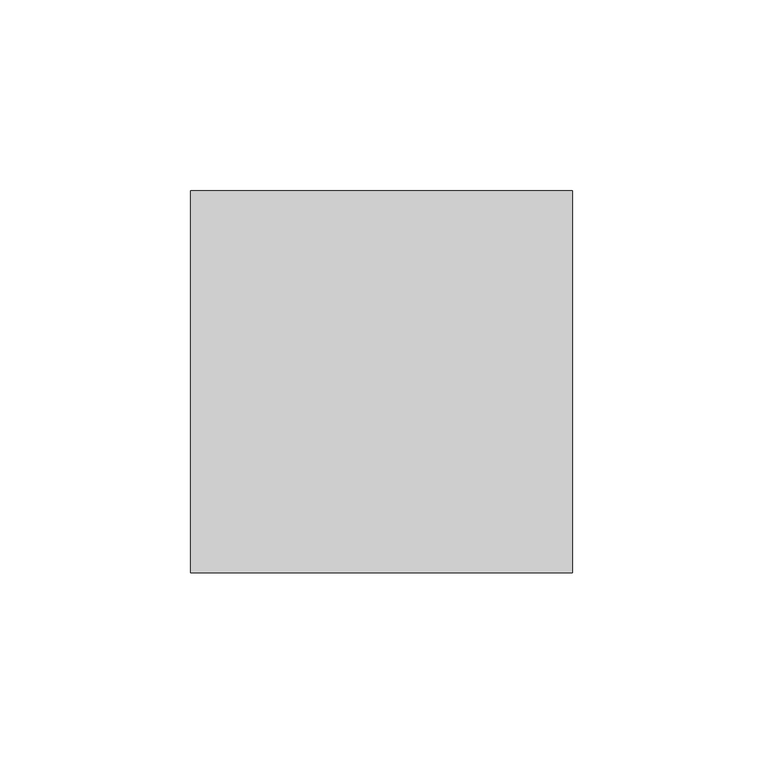
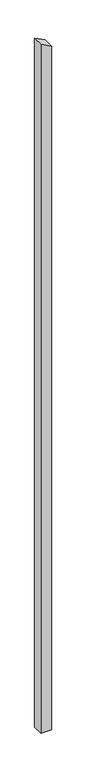
"""IFC4 building model written with IfcOpenShell, lengths in millimetres: column geometry, Holzstütze 159406 : Holzstütze 159406."""

import ifcopenshell
import ifcopenshell.guid

model = None  # the IFC model being written
_history = None  # IfcOwnerHistory: only IFC2X3 demands one
_inside = {}  # id of a spatial element -> (the spatial element, [elements in it])
_under = {}  # id of a project, library or spatial element -> (it, [spatial elements below it])
_declared = {}  # id of a project -> (the project, [libraries it declares])
_typed = {}  # id of a type object -> (the type object, [elements of that type])
_made_of = {}  # id of a material, layer set ... -> (it, [elements and type objects made of it])


def new_model(schema):
    """Start an empty IFC model of exactly this schema.

    Asked for "IFC4X3", IfcOpenShell would pick the latest addendum, in which some entities
    have other attributes; the version numbers below select the first issue.
    IFC2X3 requires an IfcOwnerHistory on every rooted entity: one is made here for all.
    """
    global model, _history
    if schema == "IFC4X3":
        model = ifcopenshell.file(schema_version=(4, 3, 0, 0))
    else:
        model = ifcopenshell.file(schema=schema)
    _inside.clear()
    _under.clear()
    _declared.clear()
    _typed.clear()
    _made_of.clear()
    _history = None
    if model.schema == "IFC2X3":
        org = make("IfcOrganization", Name="unknown")
        user = make(
            "IfcPersonAndOrganization",
            ThePerson=make("IfcPerson", FamilyName="unknown"),
            TheOrganization=org,
        )
        app = make(
            "IfcApplication",
            ApplicationDeveloper=org,
            Version="unknown",
            ApplicationFullName="unknown",
            ApplicationIdentifier="unknown",
        )
        _history = make(
            "IfcOwnerHistory",
            OwningUser=user,
            OwningApplication=app,
            ChangeAction="ADDED",
            CreationDate=0,
        )
    return model


def make(cls, **values):
    """One entity of the class cls with the attributes given. An attribute that is None is left unset."""
    return model.create_entity(
        cls, **{name: value for name, value in values.items() if value is not None}
    )


def rooted(cls, **values):
    """An entity with a GlobalId (a new one), such as an element, a storey or a relation."""
    return make(cls, GlobalId=ifcopenshell.guid.new(), OwnerHistory=_history, **values)


def si_unit(unit_type, name, prefix=None):
    """IfcSIUnit, for example si_unit("LENGTHUNIT", "METRE", prefix="MILLI")."""
    return make("IfcSIUnit", UnitType=unit_type, Prefix=prefix, Name=name)


def assignment(units):
    """IfcUnitAssignment: the units of a project."""
    return None if units is None else make("IfcUnitAssignment", Units=units)


def point(xyz):
    """IfcCartesianPoint."""
    return None if xyz is None else make("IfcCartesianPoint", Coordinates=xyz)


def direction(xyz):
    """IfcDirection."""
    return None if xyz is None else make("IfcDirection", DirectionRatios=xyz)


def frame(location, z_axis=None, x_axis=None):
    """IfcAxis2Placement3D, a coordinate frame: its origin and axes. An axis left out is left unset."""
    return make(
        "IfcAxis2Placement3D",
        Location=point(location),
        Axis=direction(z_axis),
        RefDirection=direction(x_axis),
    )


def origin():
    """The frame at (0, 0, 0) with its axes left unset."""
    return frame((0.0, 0.0, 0.0))


def place(relative_to, where):
    """IfcLocalPlacement: puts the frame where relative to a parent placement (None: the world)."""
    return make(
        "IfcLocalPlacement", PlacementRelTo=relative_to, RelativePlacement=where
    )


def context(
    kind, dimensions, precision=None, world=None, true_north=None, identifier=None
):
    """IfcGeometricRepresentationContext, for example the 3D "Model" context."""
    return make(
        "IfcGeometricRepresentationContext",
        ContextIdentifier=identifier,
        ContextType=kind,
        CoordinateSpaceDimension=dimensions,
        Precision=precision,
        WorldCoordinateSystem=world,
        TrueNorth=true_north,
    )


def project(units=None, contexts=None):
    """IfcProject with its units and contexts."""
    return rooted(
        "IfcProject",
        Name="project",
        RepresentationContexts=contexts,
        UnitsInContext=assignment(units),
    )


def spatial(cls, under=None, at=None, **own):
    """A site, building, storey or space (cls), placed at a placement, below another one or the project."""
    s = rooted(cls, ObjectPlacement=at, **own)
    if under is not None:
        _under.setdefault(under.id(), (under, []))[1].append(s)
    return s


def polyline(points):
    """IfcPolyline through the points."""
    return make("IfcPolyline", Points=[point(p) for p in points])


def outline(outer, holes=None, kind="AREA"):
    """IfcArbitraryClosedProfileDef: a profile drawn as a closed curve; with holes, ...WithVoids."""
    if holes is None:
        return make("IfcArbitraryClosedProfileDef", ProfileType=kind, OuterCurve=outer)
    return make(
        "IfcArbitraryProfileDefWithVoids",
        ProfileType=kind,
        OuterCurve=outer,
        InnerCurves=holes,
    )


def extrude(swept, where, along, depth):
    """IfcExtrudedAreaSolid: the profile swept, set in the frame where, extruded along a direction by depth."""
    return make(
        "IfcExtrudedAreaSolid",
        SweptArea=swept,
        Position=where,
        ExtrudedDirection=direction(along),
        Depth=depth,
    )


def shape(context_of_items, identifier, shape_type, items):
    """IfcShapeRepresentation: the items that make up one representation, for example the "Body"."""
    return make(
        "IfcShapeRepresentation",
        ContextOfItems=context_of_items,
        RepresentationIdentifier=identifier,
        RepresentationType=shape_type,
        Items=items,
    )


def source(mapping_origin, context_of_items, identifier, shape_type, items):
    """IfcRepresentationMap: a shape defined once, which mapped items show again and again."""
    return make(
        "IfcRepresentationMap",
        MappingOrigin=mapping_origin,
        MappedRepresentation=shape(context_of_items, identifier, shape_type, items),
    )


def transform(
    local_origin,
    x_axis=None,
    y_axis=None,
    z_axis=None,
    scale=None,
    scale2=None,
    scale3=None,
    uniform=True,
):
    """IfcCartesianTransformationOperator3D, or its non-uniform kind. x_axis, y_axis, z_axis: its Axis1, 2, 3."""
    if uniform:
        return make(
            "IfcCartesianTransformationOperator3D",
            Axis1=direction(x_axis),
            Axis2=direction(y_axis),
            LocalOrigin=point(local_origin),
            Scale=scale,
            Axis3=direction(z_axis),
        )
    return make(
        "IfcCartesianTransformationOperator3DnonUniform",
        Axis1=direction(x_axis),
        Axis2=direction(y_axis),
        LocalOrigin=point(local_origin),
        Scale=scale,
        Axis3=direction(z_axis),
        Scale2=scale2,
        Scale3=scale3,
    )


def mapped(mapping_source, mapping_target):
    """IfcMappedItem: shows the shape of a source again, moved by a transform."""
    return make(
        "IfcMappedItem", MappingSource=mapping_source, MappingTarget=mapping_target
    )


def made_of(thing, what):
    """Note that an element or type object is made of a material, layer set ...; save() writes the relation."""
    if what is not None:
        _made_of.setdefault(what.id(), (what, []))[1].append(thing)
    return thing


def element(
    cls,
    number,
    at=None,
    inside=None,
    cuts=None,
    type_object=None,
    material=None,
    context=None,
    identifier="Body",
    shape_type=None,
    held_by="IfcProductDefinitionShape",
    body=None,
    shapes=None,
    **own,
):
    """One element of the class cls, such as IfcWall. Its Tag is "e" and its number.

    at: its placement. inside: the storey or other place that contains it. cuts: it is an
    opening in that element (IfcRelVoidsElement). A single representation is given by context,
    identifier, shape_type and body (its items); several are given by shapes. held_by: the class
    of the entity that holds the representations. save() writes the other relations.
    """
    e = rooted(cls, Tag="e%d" % number, ObjectPlacement=at, **own)
    if body is not None:
        shapes = [shape(context, identifier, shape_type, body)]
    if shapes is not None:
        e.Representation = make(held_by, Representations=shapes)
    if inside is not None:
        _inside.setdefault(inside.id(), (inside, []))[1].append(e)
    if cuts is not None:
        rooted(
            "IfcRelVoidsElement", RelatingBuildingElement=cuts, RelatedOpeningElement=e
        )
    if type_object is not None:
        _typed.setdefault(type_object.id(), (type_object, []))[1].append(e)
    return made_of(e, material)


def aggregate(whole, parts):
    """IfcRelAggregates: a whole, such as a stair, and the parts it consists of."""
    return rooted("IfcRelAggregates", RelatingObject=whole, RelatedObjects=parts)


def save(model, path):
    """Write the relations noted so far, then the file.

    IfcRelAggregates (storeys below a building ...), IfcRelContainedInSpatialStructure (elements
    in a storey), IfcRelDefinesByType, IfcRelAssociatesMaterial and IfcRelDeclares: one each for
    every whole, place, type object, material and project.
    """
    for whole, parts in _under.values():
        aggregate(whole, parts)
    for where, things in _inside.values():
        rooted(
            "IfcRelContainedInSpatialStructure",
            RelatedElements=things,
            RelatingStructure=where,
        )
    for kind, things in _typed.values():
        rooted("IfcRelDefinesByType", RelatedObjects=things, RelatingType=kind)
    for what, things in _made_of.values():
        rooted("IfcRelAssociatesMaterial", RelatedObjects=things, RelatingMaterial=what)
    for by, libraries in _declared.values():
        rooted("IfcRelDeclares", RelatingContext=by, RelatedDefinitions=libraries)
    model.write(path)


def column_ac924ca4(model_context):
    return source(origin(), model_context, "Body", "SweptSolid", [
        extrude(outline(polyline([(-500.0, 174197.7593015), (-500.0, 174297.7593015), (6345.7118258, 174297.7593015), (6396.6643707, 174197.7593015), (-500.0, 174197.7593015)])), frame((0.0, 44151.7297978, 0.0), z_axis=(0.0, 1.0, 0.0), x_axis=(0.0, 0.0, 1.0)), (0.0, 0.0, 1.0), 100.0),
    ])


if __name__ == "__main__":
    model = new_model("IFC4")
    model_context = context("Model", 3, world=origin())
    ifc_project = project(units=[si_unit("LENGTHUNIT", "METRE", prefix="MILLI")], contexts=[model_context])
    site = spatial("IfcSite", under=ifc_project)
    building = spatial("IfcBuilding", under=site)
    placement = place(None, origin())
    column_shape = column_ac924ca4(model_context)
    element("IfcColumn", 1, ObjectType="Holzstütze 159406 : Holzstütze 159406", at=placement, inside=building, context=model_context, shape_type="MappedRepresentation", body=[
        mapped(column_shape, transform((0.0, 0.0, 0.0), x_axis=(1.0, 0.0, 0.0), y_axis=(0.0, 1.0, 0.0), z_axis=(0.0, 0.0, 1.0))),
    ])
    save(model, "model.ifc")

# Revit data of these elements
# Type "Holzstütze 159406 : Holzstütze 159406"
#   Abrechnungsart = "m"
#   Allright_Bauteil_ID = "0152St 0000143354"
#   Bezeichnung = "Holzstütze"
#   Codetext = "ST-HOLZ\\"
#   Gewerk = "Zimmer- und Holzbauarbeiten"
#   Material = "Holz"
#   Objektname = "Stütze"
#   NameOverride = "Holzstütze"
#   Reference = "Holzstütze"
#   Status = "NEW"
#   ThermalTransmittance = 0.0000 BTU/(h·ft²·°F)
#   Roll = 0.00°
#   Slope = 0.00°
#   2D Interaktion = yes
#   IsExternal = yes
#   LoadBearing = yes
# Element 1 (IfcColumn, "Holzstütze 159406 : Holzstütze 159406")
#   Materials on its faces: "holzschalung"
# Materials
#   "holzschalung": class "Unassigned", colour RGB 128 128 128, transparency 0
